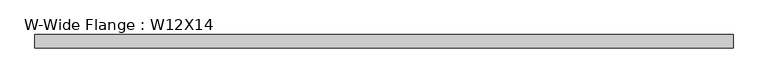
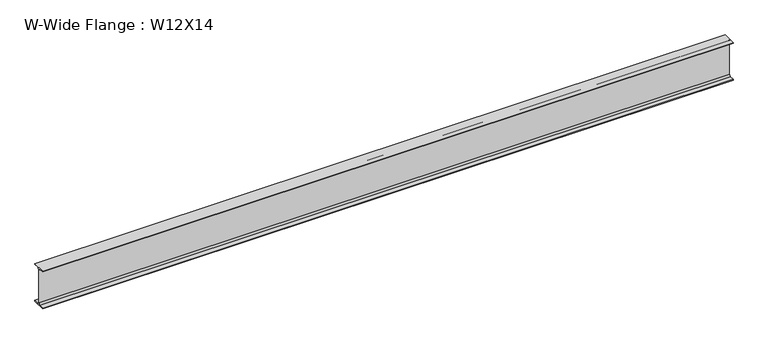
"""IFC4 building model written with IfcOpenShell, lengths in millimetres: beam geometry, W-Wide Flange : W12X14."""

from ifc_helpers import new_model, si_unit, point, frame, frame_2d, origin, place, context, project, spatial, polyline, circle_curve, trimmed, segment, composite_curve, outline, extrude, source, transform, mapped, element, save


def w_wide_flange_w12x14_81ee6899(model_context):
    return source(origin(), model_context, "Body", "SweptSolid", [
        extrude(outline(composite_curve([segment(polyline([(50.419, -145.415), (50.419, -151.13), (-50.419, -151.13), (-50.419, -145.415), (-15.875, -145.415)]), True, "CONTINUOUS"), segment(trimmed(circle_curve(frame_2d((-15.875, -132.08)), 13.335), [point((-15.875, -145.415))], [point((-2.54, -132.08))], True, "CARTESIAN"), True, "CONTINUOUS"), segment(polyline([(-2.54, -132.08), (-2.54, 132.08)]), True, "CONTINUOUS"), segment(trimmed(circle_curve(frame_2d((-15.875, 132.08)), 13.335), [point((-2.54, 132.08))], [point((-15.875, 145.415))], True, "CARTESIAN"), True, "CONTINUOUS"), segment(polyline([(-15.875, 145.415), (-50.419, 145.415), (-50.419, 151.13), (50.419, 151.13), (50.419, 145.415), (15.875, 145.415)]), True, "CONTINUOUS"), segment(trimmed(circle_curve(frame_2d((15.875, 132.08)), 13.335), [point((15.875, 145.415))], [point((2.54, 132.08))], True, "CARTESIAN"), True, "CONTINUOUS"), segment(polyline([(2.54, 132.08), (2.54, -132.08)]), True, "CONTINUOUS"), segment(trimmed(circle_curve(frame_2d((15.875, -132.08)), 13.335), [point((2.54, -132.08))], [point((15.875, -145.415))], True, "CARTESIAN"), True, "CONTINUOUS"), segment(polyline([(15.875, -145.415), (50.419, -145.415)]), True, "CONTINUOUS")], self_intersect=False)), frame((-2637.9500922, 0.0, 0.0), z_axis=(1.0, 0.0, 0.0), x_axis=(0.0, 1.0, 0.0)), (0.0, 0.0, 1.0), 5254.7910599),
    ])


if __name__ == "__main__":
    model = new_model("IFC4")
    model_context = context("Model", 3, world=origin())
    ifc_project = project(units=[si_unit("LENGTHUNIT", "METRE", prefix="MILLI")], contexts=[model_context])
    site = spatial("IfcSite", under=ifc_project)
    building = spatial("IfcBuilding", under=site)
    placement = place(None, origin())
    w_wide_flange_w12x14_shape = w_wide_flange_w12x14_81ee6899(model_context)
    element("IfcBeam", 1, ObjectType="W-Wide Flange : W12X14", at=placement, inside=building, context=model_context, shape_type="MappedRepresentation", body=[
        mapped(w_wide_flange_w12x14_shape, transform((0.0, 0.0, 0.0), x_axis=(1.0, 0.0, 0.0), y_axis=(0.0, 1.0, 0.0), z_axis=(0.0, 0.0, 1.0))),
    ])
    save(model, "model.ifc")

# Revit data of these elements
# Type "W-Wide Flange : W12X14"
#   Assembly Code = "B10"
#   W = 14
#   Length [instance default] = 5' - 0"
#   bf = 0' - 3.97"
#   d = 0' - 11.9"
#   k = 0' - 0 3/4"
#   k2 = 0' - 0.525"
#   tf = 0' - 0.225"
#   tw = 0' - 0.2"
#   A = 0.0288889 SF
#   Structural Material [instance default] = Steel ASTM A992
# Element 1 (IfcBeam, "W-Wide Flange : W12X14")
#   Materials on its faces: "Steel ASTM A992"
# Materials
#   "Steel ASTM A992": class "Metal", colour RGB 199 199 199, transparency 0, Description = "Structural steel 50ksi", Cost = 0
